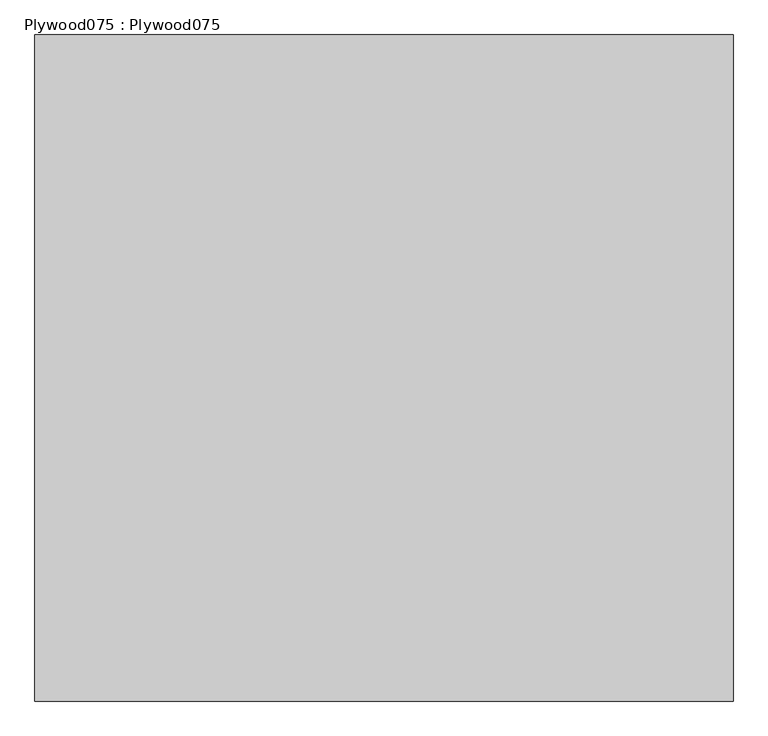
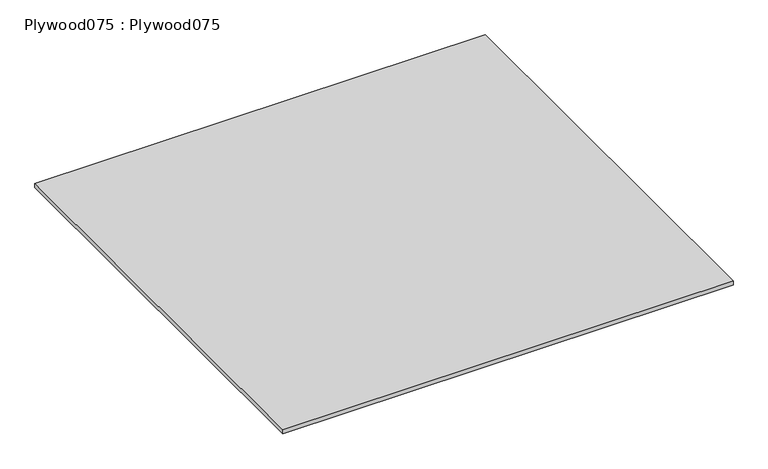
"""IFC4 building model written with IfcOpenShell, lengths in millimetres: proxy geometry, Plywood075 : Plywood075."""

from ifc_helpers import new_model, si_unit, frame, origin, place, context, project, spatial, polyline, outline, extrude, source, transform, mapped, element, save


def plywood075_plywood075_536b8c5c(model_context):
    return source(origin(), model_context, "Body", "SweptSolid", [
        extrude(outline(polyline([(-2764.2237014, 947.1093426), (-668.0864422, 947.1093426), (-668.0864422, -1052.8906574), (-2764.2237014, -1052.8906574), (-2764.2237014, 947.1093426)])), frame((0.0, 0.0, 39560.2460083), z_axis=(0.0, 0.0, 1.0), x_axis=(1.0, 0.0, 0.0)), (0.0, 0.0, 1.0), 19.05),
    ])


if __name__ == "__main__":
    model = new_model("IFC4")
    model_context = context("Model", 3, world=origin())
    ifc_project = project(units=[si_unit("LENGTHUNIT", "METRE", prefix="MILLI")], contexts=[model_context])
    site = spatial("IfcSite", under=ifc_project)
    building = spatial("IfcBuilding", under=site)
    placement = place(None, origin())
    plywood075_plywood075_shape = plywood075_plywood075_536b8c5c(model_context)
    element("IfcBuildingElementProxy", 1, Name="Plywood075 : Plywood075", ObjectType="Plywood075 : Plywood075", at=placement, inside=building, context=model_context, shape_type="MappedRepresentation", body=[
        mapped(plywood075_plywood075_shape, transform((0.0, 0.0, 0.0), x_axis=(1.0, 0.0, 0.0), y_axis=(0.0, 1.0, 0.0), z_axis=(0.0, 0.0, 1.0))),
    ])
    save(model, "model.ifc")

# Revit data of these elements
# Type "Plywood075 : Plywood075"
#   NameOverride = "Plywood075"
# Element 1 (IfcBuildingElementProxy, "Plywood075 : Plywood075")
#   Materials on its faces: "CDX PLYWOOD -  SEE STRUCTURAL DWGS"
# Materials
#   "CDX PLYWOOD -  SEE STRUCTURAL DWGS": class "Unassigned", colour RGB 177 130 114, transparency 0, Cost = 0
